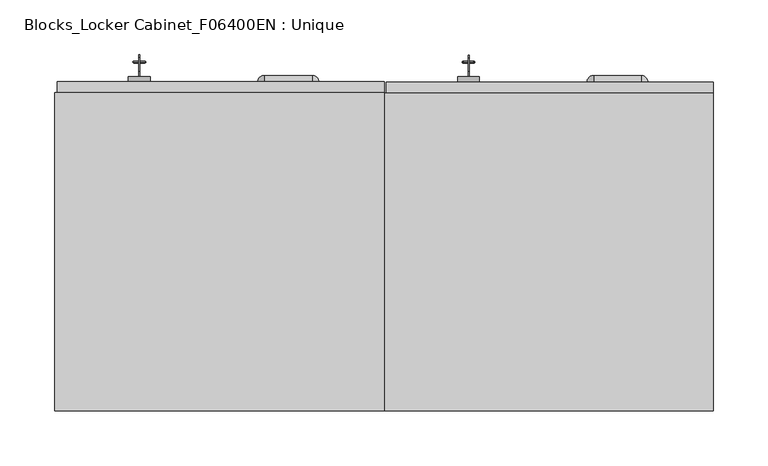
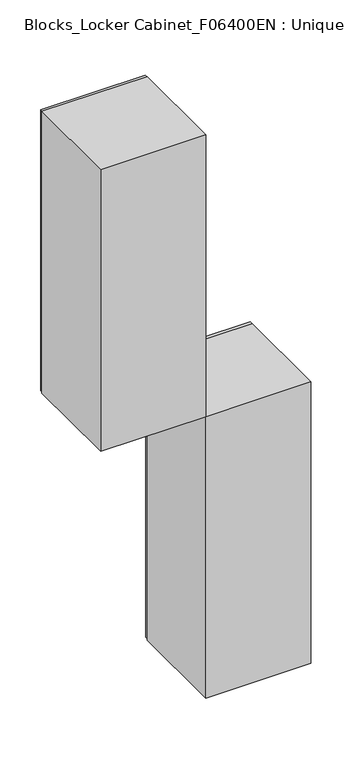
"""IFC4 building model written with IfcOpenShell, lengths in millimetres: furniture geometry, Blocks_Locker Cabinet_F06400EN : Unique."""

from ifc_helpers import new_model, si_unit, point, frame, frame_2d, origin, place, context, project, spatial, polyline, circle_curve, ellipse_curve, trimmed, segment, composite_curve, outline, extrude, faceted_brep, source, transform, mapped, element, save
from ifc_brep_helpers import plane_surface, cylinder_surface, revolved_surface, advanced_brep


def blocks_locker_cabinet_f06400en_unique_48c8ac53(model_context):
    return source(origin(), model_context, "Body", "SolidModel", [
        advanced_brep(
        [(-383.0, 12.5, 1375.0), (-363.0, 12.5, 1375.0), (-371.1588195, 12.5, 1382.0962926), (-374.8411805, 12.5, 1382.0962926), (-374.8411805, 12.5, 1372.8618188), (-371.1588195, 12.5, 1372.8618188), (-383.0, 7.5, 1375.0), (-363.0, 7.5, 1375.0), (-363.0, 10.7450625, 1375.0), (-383.0, 10.7450625, 1375.0), (-371.1588195, 10.7450625, 1372.8618188), (-371.1588195, 10.7450625, 1382.0962926), (-374.8411805, 10.7450625, 1372.8618188), (-374.8411805, 10.7450625, 1382.0962926)],
        [
            (0, 1, circle_curve(frame((-373.0, 12.5, 1375.0), z_axis=(0.0, 1.0, 0.0), x_axis=(1.0, 0.0, 0.0)), 10.0)),
            (1, 0, circle_curve(frame((-373.0, 12.5, 1375.0), z_axis=(0.0, 1.0, 0.0), x_axis=(1.0, 0.0, 0.0)), 10.0)),
            (2, 3),
            (3, 4),
            (4, 5),
            (5, 2),
            (6, 7, circle_curve(frame((-373.0, 7.5, 1375.0), z_axis=(0.0, -1.0, 0.0), x_axis=(1.0, 0.0, 0.0)), 10.0)),
            (7, 6, circle_curve(frame((-373.0, 7.5, 1375.0), z_axis=(0.0, -1.0, 0.0), x_axis=(1.0, 0.0, 0.0)), 10.0)),
            (1, 8),
            (8, 7),
            (6, 9),
            (9, 0),
            (5, 10),
            (10, 11),
            (11, 2),
            (4, 12),
            (12, 10),
            (3, 13),
            (13, 12),
            (11, 13),
        ],
        [
            plane_surface(frame((-363.0, 12.5, 1375.0), z_axis=(0.0, 1.0, 0.0), x_axis=(0.0, 0.0, 1.0))),
            plane_surface(frame((-363.0, 7.5, 1375.0), z_axis=(0.0, -1.0, 0.0), x_axis=(0.0, 0.0, -1.0))),
            cylinder_surface(frame((-373.0, 7.5, 1375.0), z_axis=(0.0, 1.0, 0.0), x_axis=(1.0, 0.0, 0.0)), 10.0),
            plane_surface(frame((-371.1588195, 12.5, 1382.0962926), z_axis=(-1.0, 0.0, 0.0), x_axis=(0.0, -1.0, 0.0))),
            plane_surface(frame((-371.1588195, 12.5, 1372.8618188), z_axis=(0.0, 0.0, 1.0), x_axis=(0.0, -1.0, 0.0))),
            plane_surface(frame((-374.8411805, 12.5, 1372.8618188), z_axis=(1.0, 0.0, 0.0), x_axis=(0.0, -1.0, 0.0))),
            plane_surface(frame((-374.8411805, 12.5, 1382.0962926), z_axis=(0.0, 0.0, -1.0), x_axis=(0.0, -1.0, 0.0))),
            plane_surface(frame((-363.0, 10.7450625, 1375.0), z_axis=(0.0, 1.0, 0.0), x_axis=(0.0, 0.0, 1.0))),
        ],
        [
            (0, [[1, 2], [3, 4, 5, 6]]),
            (1, [[7, 8]]),
            (2, [[9, 10, -7, 11, 12, -2]]),
            (2, [[-12, -11, -8, -10, -9, -1]]),
            (3, [[13, 14, 15, -6]]),
            (4, [[16, 17, -13, -5]]),
            (5, [[18, 19, -16, -4]]),
            (6, [[-15, 20, -18, -3]]),
            (7, [[-17, -19, -20, -14]]),
        ],
    ),
        extrude(outline(composite_curve([segment(polyline([(16.8246351, 1372.8618188), (13.7848488, 1372.8618188)]), True, "CONTINUOUS"), segment(trimmed(circle_curve(frame_2d((12.908516, 1372.8618188)), 0.8763328), [point((13.7848488, 1372.8618188))], [point((12.0321832, 1372.8618188))], True, "CARTESIAN"), True, "CONTINUOUS"), segment(polyline([(12.0321832, 1372.8618188), (10.7450625, 1372.8618188), (10.7450625, 1377.6669902), (17.0336838, 1377.6669902)]), True, "CONTINUOUS"), segment(trimmed(circle_curve(frame_2d((23.0067332, 1375.0)), 6.5414185), [point((17.0336838, 1377.6669902))], [point((16.8246351, 1372.8618188))], False, "CARTESIAN"), True, "CONTINUOUS")], self_intersect=False), holes=[composite_curve([segment(trimmed(circle_curve(frame_2d((25.6281997, 1375.0)), 1.688217), [point((27.3164167, 1375.0))], [point((23.9399827, 1375.0))], True, "CARTESIAN"), True, "CONTINUOUS"), segment(trimmed(circle_curve(frame_2d((25.6281997, 1375.0)), 1.688217), [point((23.9399827, 1375.0))], [point((27.3164167, 1375.0))], True, "CARTESIAN"), True, "CONTINUOUS")], self_intersect=False)]), frame((-373.4043078, 0.0, 0.0), z_axis=(1.0, 0.0, 0.0), x_axis=(0.0, 1.0, 0.0)), (0.0, 0.0, 1.0), 0.9157402),
        extrude(outline(composite_curve([segment(polyline([(27.8125, 1354.8018875), (27.8125, 1351.7621012)]), True, "CONTINUOUS"), segment(trimmed(circle_curve(frame_2d((27.8125, 1350.8857684)), 0.8763328), [point((27.8125, 1351.7621012))], [point((27.8125, 1350.0094356))], True, "CARTESIAN"), True, "CONTINUOUS"), segment(polyline([(27.8125, 1350.0094356), (27.8125, 1347.7621012)]), True, "CONTINUOUS"), segment(trimmed(circle_curve(frame_2d((27.8125, 1346.8857684)), 0.8763328), [point((27.8125, 1347.7621012))], [point((27.8125, 1346.0094356))], True, "CARTESIAN"), True, "CONTINUOUS"), segment(polyline([(27.8125, 1346.0094356), (27.8125, 1343.7621012)]), True, "CONTINUOUS"), segment(trimmed(circle_curve(frame_2d((27.8125, 1342.8857684)), 0.8763328), [point((27.8125, 1343.7621012))], [point((27.8125, 1342.0094356))], True, "CARTESIAN"), True, "CONTINUOUS"), segment(polyline([(27.8125, 1342.0094356), (27.8125, 1340.3532579), (25.9613419, 1337.7095301), (24.2573286, 1337.7095301), (24.2573286, 1354.5978839)]), True, "CONTINUOUS"), segment(trimmed(circle_curve(frame_2d((25.6743188, 1360.9839856)), 6.5414185), [point((24.2573286, 1354.5978839))], [point((27.8125, 1354.8018875))], False, "CARTESIAN"), True, "CONTINUOUS")], self_intersect=False), holes=[composite_curve([segment(trimmed(circle_curve(frame_2d((25.6743188, 1363.6054521)), 1.688217), [point((25.6743188, 1365.2936691))], [point((25.6743188, 1361.9172351))], True, "CARTESIAN"), True, "CONTINUOUS"), segment(trimmed(circle_curve(frame_2d((25.6743188, 1363.6054521)), 1.688217), [point((25.6743188, 1361.9172351))], [point((25.6743188, 1365.2936691))], True, "CARTESIAN"), True, "CONTINUOUS")], self_intersect=False)]), frame((-373.4043078, 0.0, 0.0), z_axis=(1.0, 0.0, 0.0), x_axis=(0.0, 1.0, 0.0)), (0.0, 0.0, 1.0), 0.9157402),
        advanced_brep(
        [(-368.8, 25.663019, 1369.4000012), (-367.2, 25.663019, 1369.4000012), (-378.8, 25.663019, 1369.4000012), (-377.2, 25.663019, 1369.4000012)],
        [
            (0, 1, circle_curve(frame((-368.0, 25.663019, 1369.4000012), z_axis=(0.0, 0.0, -1.0), x_axis=(-1.0, 0.0, 0.0)), 0.8)),
            (1, 2, circle_curve(frame((-373.0, 25.663019, 1369.4000012), z_axis=(0.0, 1.0, 0.0), x_axis=(-1.0, 0.0, 0.0)), 5.8)),
            (2, 3, circle_curve(frame((-378.0, 25.663019, 1369.4000012), z_axis=(0.0, 0.0, -1.0), x_axis=(1.0, 0.0, 0.0)), 0.8)),
            (3, 0, circle_curve(frame((-373.0, 25.663019, 1369.4000012), z_axis=(0.0, -1.0, 0.0), x_axis=(-1.0, 0.0, 0.0)), 4.2)),
            (1, 0, circle_curve(frame((-368.0, 25.663019, 1369.4000012), z_axis=(0.0, 0.0, -1.0), x_axis=(-1.0, 0.0, 0.0)), 0.8)),
            (3, 2, circle_curve(frame((-378.0, 25.663019, 1369.4000012), z_axis=(0.0, 0.0, -1.0), x_axis=(1.0, 0.0, 0.0)), 0.8)),
            (2, 1, circle_curve(frame((-373.0, 25.663019, 1369.4000012), z_axis=(0.0, 1.0, 0.0), x_axis=(1.0, 0.0, 0.0)), 5.8)),
            (0, 3, circle_curve(frame((-373.0, 25.663019, 1369.4000012), z_axis=(0.0, -1.0, 0.0), x_axis=(1.0, 0.0, 0.0)), 4.2)),
        ],
        [
            revolved_surface(trimmed(ellipse_curve(frame((-378.0, 25.663019, 1369.4000012), z_axis=(0.0, 0.0, -1.0), x_axis=(1.0, 0.0, 0.0)), 0.8, 0.8), [point((-378.8, 25.663019, 1369.4000012))], [point((-377.2, 25.663019, 1369.4000012))], True, "CARTESIAN"), (-373.0, -2.5, 1369.4000012), (0.0, 1.0, 0.0)),
            revolved_surface(trimmed(ellipse_curve(frame((-378.0, 25.663019, 1369.4000012), z_axis=(0.0, 0.0, -1.0), x_axis=(1.0, 0.0, 0.0)), 0.8, 0.8), [point((-377.2, 25.663019, 1369.4000012))], [point((-378.8, 25.663019, 1369.4000012))], True, "CARTESIAN"), (-373.0, -2.5, 1369.4000012), (0.0, 1.0, 0.0)),
            revolved_surface(trimmed(ellipse_curve(frame((-368.0, 25.663019, 1369.4000012), z_axis=(0.0, 0.0, 1.0), x_axis=(-1.0, 0.0, 0.0)), 0.8, 0.8), [point((-367.2, 25.663019, 1369.4000012))], [point((-368.8, 25.663019, 1369.4000012))], True, "CARTESIAN"), (-373.0, -2.5, 1369.4000012), (0.0, 1.0, 0.0)),
            revolved_surface(trimmed(ellipse_curve(frame((-368.0, 25.663019, 1369.4000012), z_axis=(0.0, 0.0, 1.0), x_axis=(-1.0, 0.0, 0.0)), 0.8, 0.8), [point((-368.8, 25.663019, 1369.4000012))], [point((-367.2, 25.663019, 1369.4000012))], True, "CARTESIAN"), (-373.0, -2.5, 1369.4000012), (0.0, 1.0, 0.0)),
        ],
        [
            (0, [[1, 2, 3, 4]]),
            (1, [[5, -4, 6, -2]]),
            (2, [[-3, 7, -1, 8]]),
            (3, [[-6, -8, -5, -7]]),
        ],
    ),
        advanced_brep(
        [(-448.0, 7.5, 1799.0), (-448.0, -2.5, 1799.0), (-150.0, -2.5, 1799.0), (-150.0, 7.5, 1799.0), (-448.0, 7.5, 951.0), (-150.0, 7.5, 951.0), (-150.0, -2.5, 951.0), (-448.0, -2.5, 951.0), (-393.0, 7.5, 1525.0), (-393.0, 7.5, 1405.0), (-333.7890736, 7.5, 1405.0), (-333.7890736, 7.5, 1525.0), (-380.6526901, 0.3712773, 1525.0), (-357.2105549, 3.975278, 1525.0), (-380.6526901, 0.3712773, 1405.0), (-357.2105549, 3.975278, 1405.0)],
        [
            (0, 1),
            (1, 2),
            (2, 3),
            (3, 0),
            (4, 5),
            (5, 6),
            (6, 7),
            (7, 4),
            (3, 5),
            (4, 0),
            (8, 9),
            (9, 10),
            (10, 11),
            (11, 8),
            (2, 6),
            (1, 7),
            (12, 8),
            (11, 13),
            (13, 12, circle_curve(frame((-371.1776523, 16.7825242, 1525.0), z_axis=(0.0, 0.0, -1.0), x_axis=(0.0, 1.0, 0.0)), 18.9500756)),
            (14, 15, circle_curve(frame((-371.1776523, 16.7825242, 1405.0), z_axis=(0.0, 0.0, 1.0), x_axis=(0.0, 1.0, 0.0)), 18.9500756)),
            (15, 10),
            (9, 14),
            (12, 14),
            (15, 13),
        ],
        [
            plane_surface(frame((-150.0, 7.5, 1799.0), z_axis=(0.0, 0.0, 1.0), x_axis=(1.0, 0.0, 0.0))),
            plane_surface(frame((-150.0, 7.5, 951.0), z_axis=(0.0, 0.0, -1.0), x_axis=(-1.0, 0.0, 0.0))),
            plane_surface(frame((-448.0, 7.5, 1799.0), z_axis=(0.0, 1.0, 0.0), x_axis=(0.0, 0.0, -1.0))),
            plane_surface(frame((-150.0, 7.5, 1799.0), z_axis=(1.0, 0.0, 0.0), x_axis=(0.0, 0.0, -1.0))),
            plane_surface(frame((-150.0, -2.5, 1799.0), z_axis=(0.0, -1.0, 0.0), x_axis=(0.0, 0.0, -1.0))),
            plane_surface(frame((-448.0, -2.5, 1799.0), z_axis=(-1.0, 0.0, 0.0), x_axis=(0.0, 0.0, -1.0))),
            plane_surface(frame((-393.0, 7.5, 1525.0), z_axis=(0.0, 0.0, -1.0), x_axis=(-0.866025403784437, 0.5000000000000028, 0.0))),
            plane_surface(frame((-393.0, 7.5, 1405.0), z_axis=(0.0, 0.0, 1.0), x_axis=(0.866025403784437, -0.5000000000000028, 0.0))),
            plane_surface(frame((-380.6526901, 0.3712773, 1525.0), z_axis=(0.5000000000000028, 0.866025403784437, 0.0), x_axis=(0.0, 0.0, -1.0))),
            plane_surface(frame((-333.7890736, 7.5, 1525.0), z_axis=(-0.14881527984319862, 0.9888650122666847, 0.0), x_axis=(0.0, 0.0, -1.0))),
            revolved_surface(polyline([(-371.1776523, 35.7325998, 1525.0), (-371.1776523, 35.7325998, 1405.0)]), (-371.1776523, 16.7825242, 1405.0), (0.0, 0.0, 1.0)),
        ],
        [
            (0, [[1, 2, 3, 4]]),
            (1, [[5, 6, 7, 8]]),
            (2, [[9, -5, 10, -4], [11, 12, 13, 14]]),
            (3, [[15, -6, -9, -3]]),
            (4, [[16, -7, -15, -2]]),
            (5, [[-10, -8, -16, -1]]),
            (6, [[17, -14, 18, 19]]),
            (7, [[20, 21, -12, 22]]),
            (8, [[23, -22, -11, -17]]),
            (9, [[-13, -21, 24, -18]]),
            (10, [[-24, -20, -23, -19]]),
        ],
    ),
        advanced_brep(
        [(-265.0, 7.5, 991.0), (-209.4810333, 7.5, 991.0), (-215.4810333, 7.5, 997.0), (-259.0, 7.5, 997.0), (-259.0, 13.5, 991.0), (-215.4810333, 13.5, 991.0)],
        [
            (0, 1),
            (1, 2, circle_curve(frame((-215.4810333, 7.5, 991.0), z_axis=(0.0, -1.0, 0.0), x_axis=(1.0, 0.0, 0.0)), 6.0)),
            (2, 3),
            (3, 0, circle_curve(frame((-259.0, 7.5, 991.0), z_axis=(0.0, -1.0, 0.0), x_axis=(1.0, 0.0, 0.0)), 6.0)),
            (0, 4, circle_curve(frame((-259.0, 7.5, 991.0), z_axis=(0.0, 0.0, -1.0), x_axis=(1.0, 0.0, 0.0)), 6.0)),
            (4, 5),
            (5, 1, circle_curve(frame((-215.4810333, 7.5, 991.0), z_axis=(0.0, 0.0, -1.0), x_axis=(1.0, 0.0, 0.0)), 6.0)),
            (3, 4, circle_curve(frame((-259.0, 7.5, 991.0), z_axis=(-1.0, 0.0, 0.0), x_axis=(0.0, 0.0, 1.0)), 6.0)),
            (2, 5, circle_curve(frame((-215.4810333, 7.5, 991.0), z_axis=(-1.0, 0.0, 0.0), x_axis=(0.0, 0.0, 1.0)), 6.0)),
        ],
        [
            plane_surface(frame((-215.0, 7.5, 991.0), z_axis=(0.0, -1.0, 0.0), x_axis=(0.0, 0.0, 1.0))),
            plane_surface(frame((-215.0, 7.5, 991.0), z_axis=(0.0, 0.0, -1.0), x_axis=(0.0, 1.0, 0.0))),
            revolved_surface(trimmed(ellipse_curve(frame((-259.0, 7.5, 991.0), z_axis=(0.0, 1.0, 0.0), x_axis=(1.0, 0.0, 0.0)), 6.0, 6.0), [point((-265.0, 7.5, 991.0))], [point((-259.0, 7.5, 997.0))], True, "CARTESIAN"), (-215.0, 7.5, 991.0), (1.0, 0.0, 0.0)),
            cylinder_surface(frame((-215.0, 7.5, 991.0), z_axis=(1.0, 0.0, 0.0), x_axis=(0.0, 0.0, 1.0)), 6.0),
            revolved_surface(trimmed(ellipse_curve(frame((-215.4810333, 7.5, 991.0), z_axis=(0.0, 1.0, 0.0), x_axis=(1.0, 0.0, 0.0)), 6.0, 6.0), [point((-215.4810333, 7.5, 997.0))], [point((-209.4810333, 7.5, 991.0))], True, "CARTESIAN"), (-215.0, 7.5, 991.0), (1.0, 0.0, 0.0)),
        ],
        [
            (0, [[1, 2, 3, 4]]),
            (1, [[-1, 5, 6, 7]]),
            (2, [[-5, -4, 8]]),
            (3, [[-6, -8, -3, 9]]),
            (4, [[-7, -9, -2]]),
        ],
    ),
        advanced_brep(
        [(-265.0, 7.5, 1006.0), (-209.4810333, 7.5, 1006.0), (-215.4810333, 7.5, 1012.0), (-259.0, 7.5, 1012.0), (-259.0, 13.5, 1006.0), (-215.4810333, 13.5, 1006.0)],
        [
            (0, 1),
            (1, 2, circle_curve(frame((-215.4810333, 7.5, 1006.0), z_axis=(0.0, -1.0, 0.0), x_axis=(1.0, 0.0, 0.0)), 6.0)),
            (2, 3),
            (3, 0, circle_curve(frame((-259.0, 7.5, 1006.0), z_axis=(0.0, -1.0, 0.0), x_axis=(1.0, 0.0, 0.0)), 6.0)),
            (0, 4, circle_curve(frame((-259.0, 7.5, 1006.0), z_axis=(0.0, 0.0, -1.0), x_axis=(1.0, 0.0, 0.0)), 6.0)),
            (4, 5),
            (5, 1, circle_curve(frame((-215.4810333, 7.5, 1006.0), z_axis=(0.0, 0.0, -1.0), x_axis=(1.0, 0.0, 0.0)), 6.0)),
            (3, 4, circle_curve(frame((-259.0, 7.5, 1006.0), z_axis=(-1.0, 0.0, 0.0), x_axis=(0.0, 0.0, 1.0)), 6.0)),
            (2, 5, circle_curve(frame((-215.4810333, 7.5, 1006.0), z_axis=(-1.0, 0.0, 0.0), x_axis=(0.0, 0.0, 1.0)), 6.0)),
        ],
        [
            plane_surface(frame((-215.0, 7.5, 1006.0), z_axis=(0.0, -1.0, 0.0), x_axis=(0.0, 0.0, 1.0))),
            plane_surface(frame((-215.0, 7.5, 1006.0), z_axis=(0.0, 0.0, -1.0), x_axis=(0.0, 1.0, 0.0))),
            revolved_surface(trimmed(ellipse_curve(frame((-259.0, 7.5, 1006.0), z_axis=(0.0, 1.0, 0.0), x_axis=(1.0, 0.0, 0.0)), 6.0, 6.0), [point((-265.0, 7.5, 1006.0))], [point((-259.0, 7.5, 1012.0))], True, "CARTESIAN"), (-215.0, 7.5, 1006.0), (1.0, 0.0, 0.0)),
            cylinder_surface(frame((-215.0, 7.5, 1006.0), z_axis=(1.0, 0.0, 0.0), x_axis=(0.0, 0.0, 1.0)), 6.0),
            revolved_surface(trimmed(ellipse_curve(frame((-215.4810333, 7.5, 1006.0), z_axis=(0.0, 1.0, 0.0), x_axis=(1.0, 0.0, 0.0)), 6.0, 6.0), [point((-215.4810333, 7.5, 1012.0))], [point((-209.4810333, 7.5, 1006.0))], True, "CARTESIAN"), (-215.0, 7.5, 1006.0), (1.0, 0.0, 0.0)),
        ],
        [
            (0, [[1, 2, 3, 4]]),
            (1, [[-1, 5, 6, 7]]),
            (2, [[-5, -4, 8]]),
            (3, [[-6, -8, -3, 9]]),
            (4, [[-7, -9, -2]]),
        ],
    ),
        advanced_brep(
        [(-265.0, 7.5, 1021.0), (-209.4810333, 7.5, 1021.0), (-215.4810333, 7.5, 1027.0), (-259.0, 7.5, 1027.0), (-259.0, 13.5, 1021.0), (-215.4810333, 13.5, 1021.0)],
        [
            (0, 1),
            (1, 2, circle_curve(frame((-215.4810333, 7.5, 1021.0), z_axis=(0.0, -1.0, 0.0), x_axis=(1.0, 0.0, 0.0)), 6.0)),
            (2, 3),
            (3, 0, circle_curve(frame((-259.0, 7.5, 1021.0), z_axis=(0.0, -1.0, 0.0), x_axis=(1.0, 0.0, 0.0)), 6.0)),
            (0, 4, circle_curve(frame((-259.0, 7.5, 1021.0), z_axis=(0.0, 0.0, -1.0), x_axis=(1.0, 0.0, 0.0)), 6.0)),
            (4, 5),
            (5, 1, circle_curve(frame((-215.4810333, 7.5, 1021.0), z_axis=(0.0, 0.0, -1.0), x_axis=(1.0, 0.0, 0.0)), 6.0)),
            (3, 4, circle_curve(frame((-259.0, 7.5, 1021.0), z_axis=(-1.0, 0.0, 0.0), x_axis=(0.0, 0.0, 1.0)), 6.0)),
            (2, 5, circle_curve(frame((-215.4810333, 7.5, 1021.0), z_axis=(-1.0, 0.0, 0.0), x_axis=(0.0, 0.0, 1.0)), 6.0)),
        ],
        [
            plane_surface(frame((-215.0, 7.5, 1021.0), z_axis=(0.0, -1.0, 0.0), x_axis=(0.0, 0.0, 1.0))),
            plane_surface(frame((-215.0, 7.5, 1021.0), z_axis=(0.0, 0.0, -1.0), x_axis=(0.0, 1.0, 0.0))),
            revolved_surface(trimmed(ellipse_curve(frame((-259.0, 7.5, 1021.0), z_axis=(0.0, 1.0, 0.0), x_axis=(1.0, 0.0, 0.0)), 6.0, 6.0), [point((-265.0, 7.5, 1021.0))], [point((-259.0, 7.5, 1027.0))], True, "CARTESIAN"), (-215.0, 7.5, 1021.0), (1.0, 0.0, 0.0)),
            cylinder_surface(frame((-215.0, 7.5, 1021.0), z_axis=(1.0, 0.0, 0.0), x_axis=(0.0, 0.0, 1.0)), 6.0),
            revolved_surface(trimmed(ellipse_curve(frame((-215.4810333, 7.5, 1021.0), z_axis=(0.0, 1.0, 0.0), x_axis=(1.0, 0.0, 0.0)), 6.0, 6.0), [point((-215.4810333, 7.5, 1027.0))], [point((-209.4810333, 7.5, 1021.0))], True, "CARTESIAN"), (-215.0, 7.5, 1021.0), (1.0, 0.0, 0.0)),
        ],
        [
            (0, [[1, 2, 3, 4]]),
            (1, [[-1, 5, 6, 7]]),
            (2, [[-5, -4, 8]]),
            (3, [[-6, -8, -3, 9]]),
            (4, [[-7, -9, -2]]),
        ],
    ),
        advanced_brep(
        [(-265.0, 7.5, 1036.0), (-209.4810333, 7.5, 1036.0), (-215.4810333, 7.5, 1042.0), (-259.0, 7.5, 1042.0), (-259.0, 13.5, 1036.0), (-215.4810333, 13.5, 1036.0)],
        [
            (0, 1),
            (1, 2, circle_curve(frame((-215.4810333, 7.5, 1036.0), z_axis=(0.0, -1.0, 0.0), x_axis=(1.0, 0.0, 0.0)), 6.0)),
            (2, 3),
            (3, 0, circle_curve(frame((-259.0, 7.5, 1036.0), z_axis=(0.0, -1.0, 0.0), x_axis=(1.0, 0.0, 0.0)), 6.0)),
            (0, 4, circle_curve(frame((-259.0, 7.5, 1036.0), z_axis=(0.0, 0.0, -1.0), x_axis=(1.0, 0.0, 0.0)), 6.0)),
            (4, 5),
            (5, 1, circle_curve(frame((-215.4810333, 7.5, 1036.0), z_axis=(0.0, 0.0, -1.0), x_axis=(1.0, 0.0, 0.0)), 6.0)),
            (3, 4, circle_curve(frame((-259.0, 7.5, 1036.0), z_axis=(-1.0, 0.0, 0.0), x_axis=(0.0, 0.0, 1.0)), 6.0)),
            (2, 5, circle_curve(frame((-215.4810333, 7.5, 1036.0), z_axis=(-1.0, 0.0, 0.0), x_axis=(0.0, 0.0, 1.0)), 6.0)),
        ],
        [
            plane_surface(frame((-215.0, 7.5, 1036.0), z_axis=(0.0, -1.0, 0.0), x_axis=(0.0, 0.0, 1.0))),
            plane_surface(frame((-215.0, 7.5, 1036.0), z_axis=(0.0, 0.0, -1.0), x_axis=(0.0, 1.0, 0.0))),
            revolved_surface(trimmed(ellipse_curve(frame((-259.0, 7.5, 1036.0), z_axis=(0.0, 1.0, 0.0), x_axis=(1.0, 0.0, 0.0)), 6.0, 6.0), [point((-265.0, 7.5, 1036.0))], [point((-259.0, 7.5, 1042.0))], True, "CARTESIAN"), (-215.0, 7.5, 1036.0), (1.0, 0.0, 0.0)),
            cylinder_surface(frame((-215.0, 7.5, 1036.0), z_axis=(1.0, 0.0, 0.0), x_axis=(0.0, 0.0, 1.0)), 6.0),
            revolved_surface(trimmed(ellipse_curve(frame((-215.4810333, 7.5, 1036.0), z_axis=(0.0, 1.0, 0.0), x_axis=(1.0, 0.0, 0.0)), 6.0, 6.0), [point((-215.4810333, 7.5, 1042.0))], [point((-209.4810333, 7.5, 1036.0))], True, "CARTESIAN"), (-215.0, 7.5, 1036.0), (1.0, 0.0, 0.0)),
        ],
        [
            (0, [[1, 2, 3, 4]]),
            (1, [[-1, 5, 6, 7]]),
            (2, [[-5, -4, 8]]),
            (3, [[-6, -8, -3, 9]]),
            (4, [[-7, -9, -2]]),
        ],
    ),
        advanced_brep(
        [(-265.0, 7.5, 1051.0), (-209.4810333, 7.5, 1051.0), (-215.4810333, 7.5, 1057.0), (-259.0, 7.5, 1057.0), (-259.0, 13.5, 1051.0), (-215.4810333, 13.5, 1051.0)],
        [
            (0, 1),
            (1, 2, circle_curve(frame((-215.4810333, 7.5, 1051.0), z_axis=(0.0, -1.0, 0.0), x_axis=(1.0, 0.0, 0.0)), 6.0)),
            (2, 3),
            (3, 0, circle_curve(frame((-259.0, 7.5, 1051.0), z_axis=(0.0, -1.0, 0.0), x_axis=(1.0, 0.0, 0.0)), 6.0)),
            (0, 4, circle_curve(frame((-259.0, 7.5, 1051.0), z_axis=(0.0, 0.0, -1.0), x_axis=(1.0, 0.0, 0.0)), 6.0)),
            (4, 5),
            (5, 1, circle_curve(frame((-215.4810333, 7.5, 1051.0), z_axis=(0.0, 0.0, -1.0), x_axis=(1.0, 0.0, 0.0)), 6.0)),
            (3, 4, circle_curve(frame((-259.0, 7.5, 1051.0), z_axis=(-1.0, 0.0, 0.0), x_axis=(0.0, 0.0, 1.0)), 6.0)),
            (2, 5, circle_curve(frame((-215.4810333, 7.5, 1051.0), z_axis=(-1.0, 0.0, 0.0), x_axis=(0.0, 0.0, 1.0)), 6.0)),
        ],
        [
            plane_surface(frame((-215.0, 7.5, 1051.0), z_axis=(0.0, -1.0, 0.0), x_axis=(0.0, 0.0, 1.0))),
            plane_surface(frame((-215.0, 7.5, 1051.0), z_axis=(0.0, 0.0, -1.0), x_axis=(0.0, 1.0, 0.0))),
            revolved_surface(trimmed(ellipse_curve(frame((-259.0, 7.5, 1051.0), z_axis=(0.0, 1.0, 0.0), x_axis=(1.0, 0.0, 0.0)), 6.0, 6.0), [point((-265.0, 7.5, 1051.0))], [point((-259.0, 7.5, 1057.0))], True, "CARTESIAN"), (-215.0, 7.5, 1051.0), (1.0, 0.0, 0.0)),
            cylinder_surface(frame((-215.0, 7.5, 1051.0), z_axis=(1.0, 0.0, 0.0), x_axis=(0.0, 0.0, 1.0)), 6.0),
            revolved_surface(trimmed(ellipse_curve(frame((-215.4810333, 7.5, 1051.0), z_axis=(0.0, 1.0, 0.0), x_axis=(1.0, 0.0, 0.0)), 6.0, 6.0), [point((-215.4810333, 7.5, 1057.0))], [point((-209.4810333, 7.5, 1051.0))], True, "CARTESIAN"), (-215.0, 7.5, 1051.0), (1.0, 0.0, 0.0)),
        ],
        [
            (0, [[1, 2, 3, 4]]),
            (1, [[-1, 5, 6, 7]]),
            (2, [[-5, -4, 8]]),
            (3, [[-6, -8, -3, 9]]),
            (4, [[-7, -9, -2]]),
        ],
    ),
        extrude(outline(composite_curve([segment(polyline([(-380.6526901, 0.3712773), (-393.0, 7.5), (-333.7890736, 7.5), (-357.2105549, 3.975278)]), True, "CONTINUOUS"), segment(trimmed(circle_curve(frame_2d((-371.1776523, 16.7825242)), 18.9500756), [point((-357.2105549, 3.975278))], [point((-380.6526901, 0.3712773))], False, "CARTESIAN"), True, "CONTINUOUS")], self_intersect=False)), frame((0.0, 0.0, 1405.0), z_axis=(0.0, 0.0, 1.0), x_axis=(1.0, 0.0, 0.0)), (0.0, 0.0, 1.0), 5.0),
        extrude(outline(composite_curve([segment(polyline([(-380.6526901, 0.3712773), (-393.0, 7.5), (-333.7890736, 7.5), (-357.2105549, 3.975278)]), True, "CONTINUOUS"), segment(trimmed(circle_curve(frame_2d((-371.1776523, 16.7825242)), 18.9500756), [point((-357.2105549, 3.975278))], [point((-380.6526901, 0.3712773))], False, "CARTESIAN"), True, "CONTINUOUS")], self_intersect=False)), frame((0.0, 0.0, 1520.0), z_axis=(0.0, 0.0, 1.0), x_axis=(1.0, 0.0, 0.0)), (0.0, 0.0, 1.0), 5.0),
        faceted_brep([(-150.0, -2.5, 1800.0), (-150.0, -2.5, 950.0), (-450.0, -2.5, 950.0), (-450.0, -2.5, 1800.0), (-160.0, -2.5, 1790.0), (-440.0, -2.5, 1790.0), (-440.0, -2.5, 960.0), (-160.0, -2.5, 960.0), (-150.0, -292.5, 1800.0), (-450.0, -292.5, 1800.0), (-450.0, -292.5, 950.0), (-150.0, -292.5, 950.0), (-450.0, -282.5, 1800.0), (-150.0, -282.5, 1800.0), (-450.0, -282.5, 950.0), (-150.0, -282.5, 950.0), (-160.0, -282.5, 960.0), (-160.0, -282.5, 1790.0), (-440.0, -282.5, 960.0), (-440.0, -282.5, 1790.0)], [[[0, 1, 2, 3], [4, 5, 6, 7]], [[8, 9, 10, 11]], [[3, 12, 9, 8, 13, 0]], [[2, 14, 10, 9, 12, 3]], [[1, 15, 11, 10, 14, 2]], [[0, 13, 8, 11, 15, 1]], [[7, 16, 17, 4]], [[6, 18, 16, 7]], [[5, 19, 18, 6]], [[4, 17, 19, 5]], [[16, 18, 19, 17]]]),
        advanced_brep(
        [(-83.0, 12.5, 525.0), (-63.0, 12.5, 525.0), (-71.1588195, 12.5, 532.0962926), (-74.8411805, 12.5, 532.0962926), (-74.8411805, 12.5, 522.8618188), (-71.1588195, 12.5, 522.8618188), (-83.0, 7.5, 525.0), (-63.0, 7.5, 525.0), (-63.0, 10.7450625, 525.0), (-83.0, 10.7450625, 525.0), (-71.1588195, 10.7450625, 522.8618188), (-71.1588195, 10.7450625, 532.0962926), (-74.8411805, 10.7450625, 522.8618188), (-74.8411805, 10.7450625, 532.0962926)],
        [
            (0, 1, circle_curve(frame((-73.0, 12.5, 525.0), z_axis=(0.0, 1.0, 0.0), x_axis=(1.0, 0.0, 0.0)), 10.0)),
            (1, 0, circle_curve(frame((-73.0, 12.5, 525.0), z_axis=(0.0, 1.0, 0.0), x_axis=(1.0, 0.0, 0.0)), 10.0)),
            (2, 3),
            (3, 4),
            (4, 5),
            (5, 2),
            (6, 7, circle_curve(frame((-73.0, 7.5, 525.0), z_axis=(0.0, -1.0, 0.0), x_axis=(1.0, 0.0, 0.0)), 10.0)),
            (7, 6, circle_curve(frame((-73.0, 7.5, 525.0), z_axis=(0.0, -1.0, 0.0), x_axis=(1.0, 0.0, 0.0)), 10.0)),
            (1, 8),
            (8, 7),
            (6, 9),
            (9, 0),
            (5, 10),
            (10, 11),
            (11, 2),
            (4, 12),
            (12, 10),
            (3, 13),
            (13, 12),
            (11, 13),
        ],
        [
            plane_surface(frame((-63.0, 12.5, 525.0), z_axis=(0.0, 1.0, 0.0), x_axis=(0.0, 0.0, 1.0))),
            plane_surface(frame((-63.0, 7.5, 525.0), z_axis=(0.0, -1.0, 0.0), x_axis=(0.0, 0.0, -1.0))),
            cylinder_surface(frame((-73.0, 7.5, 525.0), z_axis=(0.0, 1.0, 0.0), x_axis=(1.0, 0.0, 0.0)), 10.0),
            plane_surface(frame((-71.1588195, 12.5, 532.0962926), z_axis=(-1.0, 0.0, 0.0), x_axis=(0.0, -1.0, 0.0))),
            plane_surface(frame((-71.1588195, 12.5, 522.8618188), z_axis=(0.0, 0.0, 1.0), x_axis=(0.0, -1.0, 0.0))),
            plane_surface(frame((-74.8411805, 12.5, 522.8618188), z_axis=(1.0, 0.0, 0.0), x_axis=(0.0, -1.0, 0.0))),
            plane_surface(frame((-74.8411805, 12.5, 532.0962926), z_axis=(0.0, 0.0, -1.0), x_axis=(0.0, -1.0, 0.0))),
            plane_surface(frame((-63.0, 10.7450625, 525.0), z_axis=(0.0, 1.0, 0.0), x_axis=(0.0, 0.0, 1.0))),
        ],
        [
            (0, [[1, 2], [3, 4, 5, 6]]),
            (1, [[7, 8]]),
            (2, [[9, 10, -7, 11, 12, -2]]),
            (2, [[-12, -11, -8, -10, -9, -1]]),
            (3, [[13, 14, 15, -6]]),
            (4, [[16, 17, -13, -5]]),
            (5, [[18, 19, -16, -4]]),
            (6, [[-15, 20, -18, -3]]),
            (7, [[-17, -19, -20, -14]]),
        ],
    ),
        extrude(outline(composite_curve([segment(polyline([(16.8246351, 522.8618188), (13.7848488, 522.8618188)]), True, "CONTINUOUS"), segment(trimmed(circle_curve(frame_2d((12.908516, 522.8618188)), 0.8763328), [point((13.7848488, 522.8618188))], [point((12.0321832, 522.8618188))], True, "CARTESIAN"), True, "CONTINUOUS"), segment(polyline([(12.0321832, 522.8618188), (10.7450625, 522.8618188), (10.7450625, 527.6669902), (17.0336838, 527.6669902)]), True, "CONTINUOUS"), segment(trimmed(circle_curve(frame_2d((23.0067332, 525.0)), 6.5414185), [point((17.0336838, 527.6669902))], [point((16.8246351, 522.8618188))], False, "CARTESIAN"), True, "CONTINUOUS")], self_intersect=False), holes=[composite_curve([segment(trimmed(circle_curve(frame_2d((25.6281997, 525.0)), 1.688217), [point((27.3164167, 525.0))], [point((23.9399827, 525.0))], True, "CARTESIAN"), True, "CONTINUOUS"), segment(trimmed(circle_curve(frame_2d((25.6281997, 525.0)), 1.688217), [point((23.9399827, 525.0))], [point((27.3164167, 525.0))], True, "CARTESIAN"), True, "CONTINUOUS")], self_intersect=False)]), frame((-73.4043078, 0.0, 0.0), z_axis=(1.0, 0.0, 0.0), x_axis=(0.0, 1.0, 0.0)), (0.0, 0.0, 1.0), 0.9157402),
        extrude(outline(composite_curve([segment(polyline([(27.8125, 504.8018875), (27.8125, 501.7621012)]), True, "CONTINUOUS"), segment(trimmed(circle_curve(frame_2d((27.8125, 500.8857684)), 0.8763328), [point((27.8125, 501.7621012))], [point((27.8125, 500.0094356))], True, "CARTESIAN"), True, "CONTINUOUS"), segment(polyline([(27.8125, 500.0094356), (27.8125, 497.7621012)]), True, "CONTINUOUS"), segment(trimmed(circle_curve(frame_2d((27.8125, 496.8857684)), 0.8763328), [point((27.8125, 497.7621012))], [point((27.8125, 496.0094356))], True, "CARTESIAN"), True, "CONTINUOUS"), segment(polyline([(27.8125, 496.0094356), (27.8125, 493.7621012)]), True, "CONTINUOUS"), segment(trimmed(circle_curve(frame_2d((27.8125, 492.8857684)), 0.8763328), [point((27.8125, 493.7621012))], [point((27.8125, 492.0094356))], True, "CARTESIAN"), True, "CONTINUOUS"), segment(polyline([(27.8125, 492.0094356), (27.8125, 490.3532579), (25.9613419, 487.7095301), (24.2573286, 487.7095301), (24.2573286, 504.5978839)]), True, "CONTINUOUS"), segment(trimmed(circle_curve(frame_2d((25.6743188, 510.9839856)), 6.5414185), [point((24.2573286, 504.5978839))], [point((27.8125, 504.8018875))], False, "CARTESIAN"), True, "CONTINUOUS")], self_intersect=False), holes=[composite_curve([segment(trimmed(circle_curve(frame_2d((25.6743188, 513.6054521)), 1.688217), [point((25.6743188, 515.2936691))], [point((25.6743188, 511.9172351))], True, "CARTESIAN"), True, "CONTINUOUS"), segment(trimmed(circle_curve(frame_2d((25.6743188, 513.6054521)), 1.688217), [point((25.6743188, 511.9172351))], [point((25.6743188, 515.2936691))], True, "CARTESIAN"), True, "CONTINUOUS")], self_intersect=False)]), frame((-73.4043078, 0.0, 0.0), z_axis=(1.0, 0.0, 0.0), x_axis=(0.0, 1.0, 0.0)), (0.0, 0.0, 1.0), 0.9157402),
        advanced_brep(
        [(-68.8, 25.663019, 519.4000012), (-67.2, 25.663019, 519.4000012), (-78.8, 25.663019, 519.4000012), (-77.2, 25.663019, 519.4000012)],
        [
            (0, 1, circle_curve(frame((-68.0, 25.663019, 519.4000012), z_axis=(0.0, 0.0, -1.0), x_axis=(-1.0, 0.0, 0.0)), 0.8)),
            (1, 2, circle_curve(frame((-73.0, 25.663019, 519.4000012), z_axis=(0.0, 1.0, 0.0), x_axis=(-1.0, 0.0, 0.0)), 5.8)),
            (2, 3, circle_curve(frame((-78.0, 25.663019, 519.4000012), z_axis=(0.0, 0.0, -1.0), x_axis=(1.0, 0.0, 0.0)), 0.8)),
            (3, 0, circle_curve(frame((-73.0, 25.663019, 519.4000012), z_axis=(0.0, -1.0, 0.0), x_axis=(-1.0, 0.0, 0.0)), 4.2)),
            (1, 0, circle_curve(frame((-68.0, 25.663019, 519.4000012), z_axis=(0.0, 0.0, -1.0), x_axis=(-1.0, 0.0, 0.0)), 0.8)),
            (3, 2, circle_curve(frame((-78.0, 25.663019, 519.4000012), z_axis=(0.0, 0.0, -1.0), x_axis=(1.0, 0.0, 0.0)), 0.8)),
            (2, 1, circle_curve(frame((-73.0, 25.663019, 519.4000012), z_axis=(0.0, 1.0, 0.0), x_axis=(1.0, 0.0, 0.0)), 5.8)),
            (0, 3, circle_curve(frame((-73.0, 25.663019, 519.4000012), z_axis=(0.0, -1.0, 0.0), x_axis=(1.0, 0.0, 0.0)), 4.2)),
        ],
        [
            revolved_surface(trimmed(ellipse_curve(frame((-78.0, 25.663019, 519.4000012), z_axis=(0.0, 0.0, -1.0), x_axis=(1.0, 0.0, 0.0)), 0.8, 0.8), [point((-78.8, 25.663019, 519.4000012))], [point((-77.2, 25.663019, 519.4000012))], True, "CARTESIAN"), (-73.0, -2.5, 519.4000012), (0.0, 1.0, 0.0)),
            revolved_surface(trimmed(ellipse_curve(frame((-78.0, 25.663019, 519.4000012), z_axis=(0.0, 0.0, -1.0), x_axis=(1.0, 0.0, 0.0)), 0.8, 0.8), [point((-77.2, 25.663019, 519.4000012))], [point((-78.8, 25.663019, 519.4000012))], True, "CARTESIAN"), (-73.0, -2.5, 519.4000012), (0.0, 1.0, 0.0)),
            revolved_surface(trimmed(ellipse_curve(frame((-68.0, 25.663019, 519.4000012), z_axis=(0.0, 0.0, 1.0), x_axis=(-1.0, 0.0, 0.0)), 0.8, 0.8), [point((-67.2, 25.663019, 519.4000012))], [point((-68.8, 25.663019, 519.4000012))], True, "CARTESIAN"), (-73.0, -2.5, 519.4000012), (0.0, 1.0, 0.0)),
            revolved_surface(trimmed(ellipse_curve(frame((-68.0, 25.663019, 519.4000012), z_axis=(0.0, 0.0, 1.0), x_axis=(-1.0, 0.0, 0.0)), 0.8, 0.8), [point((-68.8, 25.663019, 519.4000012))], [point((-67.2, 25.663019, 519.4000012))], True, "CARTESIAN"), (-73.0, -2.5, 519.4000012), (0.0, 1.0, 0.0)),
        ],
        [
            (0, [[1, 2, 3, 4]]),
            (1, [[5, -4, 6, -2]]),
            (2, [[-3, 7, -1, 8]]),
            (3, [[-6, -8, -5, -7]]),
        ],
    ),
        advanced_brep(
        [(-148.0, 7.5, 949.0), (-148.0, -2.5, 949.0), (150.0, -2.5, 949.0), (150.0, 7.5, 949.0), (-148.0, 7.5, 101.0), (150.0, 7.5, 101.0), (150.0, -2.5, 101.0), (-148.0, -2.5, 101.0), (-93.0, 7.5, 675.0), (-93.0, 7.5, 555.0), (-33.7890736, 7.5, 555.0), (-33.7890736, 7.5, 675.0), (-80.6526901, 0.3712773, 675.0), (-57.2105549, 3.975278, 675.0), (-80.6526901, 0.3712773, 555.0), (-57.2105549, 3.975278, 555.0)],
        [
            (0, 1),
            (1, 2),
            (2, 3),
            (3, 0),
            (4, 5),
            (5, 6),
            (6, 7),
            (7, 4),
            (3, 5),
            (4, 0),
            (8, 9),
            (9, 10),
            (10, 11),
            (11, 8),
            (2, 6),
            (1, 7),
            (12, 8),
            (11, 13),
            (13, 12, circle_curve(frame((-71.1776523, 16.7825242, 675.0), z_axis=(0.0, 0.0, -1.0), x_axis=(0.0, 1.0, 0.0)), 18.9500756)),
            (14, 15, circle_curve(frame((-71.1776523, 16.7825242, 555.0), z_axis=(0.0, 0.0, 1.0), x_axis=(0.0, 1.0, 0.0)), 18.9500756)),
            (15, 10),
            (9, 14),
            (12, 14),
            (15, 13),
        ],
        [
            plane_surface(frame((150.0, 7.5, 949.0), z_axis=(0.0, 0.0, 1.0), x_axis=(1.0, 0.0, 0.0))),
            plane_surface(frame((150.0, 7.5, 101.0), z_axis=(0.0, 0.0, -1.0), x_axis=(-1.0, 0.0, 0.0))),
            plane_surface(frame((-148.0, 7.5, 949.0), z_axis=(0.0, 1.0, 0.0), x_axis=(0.0, 0.0, -1.0))),
            plane_surface(frame((150.0, 7.5, 949.0), z_axis=(1.0, 0.0, 0.0), x_axis=(0.0, 0.0, -1.0))),
            plane_surface(frame((150.0, -2.5, 949.0), z_axis=(0.0, -1.0, 0.0), x_axis=(0.0, 0.0, -1.0))),
            plane_surface(frame((-148.0, -2.5, 949.0), z_axis=(-1.0, 0.0, 0.0), x_axis=(0.0, 0.0, -1.0))),
            plane_surface(frame((-93.0, 7.5, 675.0), z_axis=(0.0, 0.0, -1.0), x_axis=(-0.866025403784437, 0.5000000000000028, 0.0))),
            plane_surface(frame((-93.0, 7.5, 555.0), z_axis=(0.0, 0.0, 1.0), x_axis=(0.866025403784437, -0.5000000000000028, 0.0))),
            plane_surface(frame((-80.6526901, 0.3712773, 675.0), z_axis=(0.5000000000000028, 0.866025403784437, 0.0), x_axis=(0.0, 0.0, -1.0))),
            plane_surface(frame((-33.7890736, 7.5, 675.0), z_axis=(-0.14881527984319862, 0.9888650122666847, 0.0), x_axis=(0.0, 0.0, -1.0))),
            revolved_surface(polyline([(-71.1776523, 35.7325998, 675.0), (-71.1776523, 35.7325998, 555.0)]), (-71.1776523, 16.7825242, 555.0), (0.0, 0.0, 1.0)),
        ],
        [
            (0, [[1, 2, 3, 4]]),
            (1, [[5, 6, 7, 8]]),
            (2, [[9, -5, 10, -4], [11, 12, 13, 14]]),
            (3, [[15, -6, -9, -3]]),
            (4, [[16, -7, -15, -2]]),
            (5, [[-10, -8, -16, -1]]),
            (6, [[17, -14, 18, 19]]),
            (7, [[20, 21, -12, 22]]),
            (8, [[23, -22, -11, -17]]),
            (9, [[-13, -21, 24, -18]]),
            (10, [[-24, -20, -23, -19]]),
        ],
    ),
        advanced_brep(
        [(35.0, 7.5, 141.0), (90.5189667, 7.5, 141.0), (84.5189667, 7.5, 147.0), (41.0, 7.5, 147.0), (41.0, 13.5, 141.0), (84.5189667, 13.5, 141.0)],
        [
            (0, 1),
            (1, 2, circle_curve(frame((84.5189667, 7.5, 141.0), z_axis=(0.0, -1.0, 0.0), x_axis=(1.0, 0.0, 0.0)), 6.0)),
            (2, 3),
            (3, 0, circle_curve(frame((41.0, 7.5, 141.0), z_axis=(0.0, -1.0, 0.0), x_axis=(1.0, 0.0, 0.0)), 6.0)),
            (0, 4, circle_curve(frame((41.0, 7.5, 141.0), z_axis=(0.0, 0.0, -1.0), x_axis=(1.0, 0.0, 0.0)), 6.0)),
            (4, 5),
            (5, 1, circle_curve(frame((84.5189667, 7.5, 141.0), z_axis=(0.0, 0.0, -1.0), x_axis=(1.0, 0.0, 0.0)), 6.0)),
            (3, 4, circle_curve(frame((41.0, 7.5, 141.0), z_axis=(-1.0, 0.0, 0.0), x_axis=(0.0, 0.0, 1.0)), 6.0)),
            (2, 5, circle_curve(frame((84.5189667, 7.5, 141.0), z_axis=(-1.0, 0.0, 0.0), x_axis=(0.0, 0.0, 1.0)), 6.0)),
        ],
        [
            plane_surface(frame((85.0, 7.5, 141.0), z_axis=(0.0, -1.0, 0.0), x_axis=(0.0, 0.0, 1.0))),
            plane_surface(frame((85.0, 7.5, 141.0), z_axis=(0.0, 0.0, -1.0), x_axis=(0.0, 1.0, 0.0))),
            revolved_surface(trimmed(ellipse_curve(frame((41.0, 7.5, 141.0), z_axis=(0.0, 1.0, 0.0), x_axis=(1.0, 0.0, 0.0)), 6.0, 6.0), [point((35.0, 7.5, 141.0))], [point((41.0, 7.5, 147.0))], True, "CARTESIAN"), (85.0, 7.5, 141.0), (1.0, 0.0, 0.0)),
            cylinder_surface(frame((85.0, 7.5, 141.0), z_axis=(1.0, 0.0, 0.0), x_axis=(0.0, 0.0, 1.0)), 6.0),
            revolved_surface(trimmed(ellipse_curve(frame((84.5189667, 7.5, 141.0), z_axis=(0.0, 1.0, 0.0), x_axis=(1.0, 0.0, 0.0)), 6.0, 6.0), [point((84.5189667, 7.5, 147.0))], [point((90.5189667, 7.5, 141.0))], True, "CARTESIAN"), (85.0, 7.5, 141.0), (1.0, 0.0, 0.0)),
        ],
        [
            (0, [[1, 2, 3, 4]]),
            (1, [[-1, 5, 6, 7]]),
            (2, [[-5, -4, 8]]),
            (3, [[-6, -8, -3, 9]]),
            (4, [[-7, -9, -2]]),
        ],
    ),
        advanced_brep(
        [(35.0, 7.5, 156.0), (90.5189667, 7.5, 156.0), (84.5189667, 7.5, 162.0), (41.0, 7.5, 162.0), (41.0, 13.5, 156.0), (84.5189667, 13.5, 156.0)],
        [
            (0, 1),
            (1, 2, circle_curve(frame((84.5189667, 7.5, 156.0), z_axis=(0.0, -1.0, 0.0), x_axis=(1.0, 0.0, 0.0)), 6.0)),
            (2, 3),
            (3, 0, circle_curve(frame((41.0, 7.5, 156.0), z_axis=(0.0, -1.0, 0.0), x_axis=(1.0, 0.0, 0.0)), 6.0)),
            (0, 4, circle_curve(frame((41.0, 7.5, 156.0), z_axis=(0.0, 0.0, -1.0), x_axis=(1.0, 0.0, 0.0)), 6.0)),
            (4, 5),
            (5, 1, circle_curve(frame((84.5189667, 7.5, 156.0), z_axis=(0.0, 0.0, -1.0), x_axis=(1.0, 0.0, 0.0)), 6.0)),
            (3, 4, circle_curve(frame((41.0, 7.5, 156.0), z_axis=(-1.0, 0.0, 0.0), x_axis=(0.0, 0.0, 1.0)), 6.0)),
            (2, 5, circle_curve(frame((84.5189667, 7.5, 156.0), z_axis=(-1.0, 0.0, 0.0), x_axis=(0.0, 0.0, 1.0)), 6.0)),
        ],
        [
            plane_surface(frame((85.0, 7.5, 156.0), z_axis=(0.0, -1.0, 0.0), x_axis=(0.0, 0.0, 1.0))),
            plane_surface(frame((85.0, 7.5, 156.0), z_axis=(0.0, 0.0, -1.0), x_axis=(0.0, 1.0, 0.0))),
            revolved_surface(trimmed(ellipse_curve(frame((41.0, 7.5, 156.0), z_axis=(0.0, 1.0, 0.0), x_axis=(1.0, 0.0, 0.0)), 6.0, 6.0), [point((35.0, 7.5, 156.0))], [point((41.0, 7.5, 162.0))], True, "CARTESIAN"), (85.0, 7.5, 156.0), (1.0, 0.0, 0.0)),
            cylinder_surface(frame((85.0, 7.5, 156.0), z_axis=(1.0, 0.0, 0.0), x_axis=(0.0, 0.0, 1.0)), 6.0),
            revolved_surface(trimmed(ellipse_curve(frame((84.5189667, 7.5, 156.0), z_axis=(0.0, 1.0, 0.0), x_axis=(1.0, 0.0, 0.0)), 6.0, 6.0), [point((84.5189667, 7.5, 162.0))], [point((90.5189667, 7.5, 156.0))], True, "CARTESIAN"), (85.0, 7.5, 156.0), (1.0, 0.0, 0.0)),
        ],
        [
            (0, [[1, 2, 3, 4]]),
            (1, [[-1, 5, 6, 7]]),
            (2, [[-5, -4, 8]]),
            (3, [[-6, -8, -3, 9]]),
            (4, [[-7, -9, -2]]),
        ],
    ),
        advanced_brep(
        [(35.0, 7.5, 171.0), (90.5189667, 7.5, 171.0), (84.5189667, 7.5, 177.0), (41.0, 7.5, 177.0), (41.0, 13.5, 171.0), (84.5189667, 13.5, 171.0)],
        [
            (0, 1),
            (1, 2, circle_curve(frame((84.5189667, 7.5, 171.0), z_axis=(0.0, -1.0, 0.0), x_axis=(1.0, 0.0, 0.0)), 6.0)),
            (2, 3),
            (3, 0, circle_curve(frame((41.0, 7.5, 171.0), z_axis=(0.0, -1.0, 0.0), x_axis=(1.0, 0.0, 0.0)), 6.0)),
            (0, 4, circle_curve(frame((41.0, 7.5, 171.0), z_axis=(0.0, 0.0, -1.0), x_axis=(1.0, 0.0, 0.0)), 6.0)),
            (4, 5),
            (5, 1, circle_curve(frame((84.5189667, 7.5, 171.0), z_axis=(0.0, 0.0, -1.0), x_axis=(1.0, 0.0, 0.0)), 6.0)),
            (3, 4, circle_curve(frame((41.0, 7.5, 171.0), z_axis=(-1.0, 0.0, 0.0), x_axis=(0.0, 0.0, 1.0)), 6.0)),
            (2, 5, circle_curve(frame((84.5189667, 7.5, 171.0), z_axis=(-1.0, 0.0, 0.0), x_axis=(0.0, 0.0, 1.0)), 6.0)),
        ],
        [
            plane_surface(frame((85.0, 7.5, 171.0), z_axis=(0.0, -1.0, 0.0), x_axis=(0.0, 0.0, 1.0))),
            plane_surface(frame((85.0, 7.5, 171.0), z_axis=(0.0, 0.0, -1.0), x_axis=(0.0, 1.0, 0.0))),
            revolved_surface(trimmed(ellipse_curve(frame((41.0, 7.5, 171.0), z_axis=(0.0, 1.0, 0.0), x_axis=(1.0, 0.0, 0.0)), 6.0, 6.0), [point((35.0, 7.5, 171.0))], [point((41.0, 7.5, 177.0))], True, "CARTESIAN"), (85.0, 7.5, 171.0), (1.0, 0.0, 0.0)),
            cylinder_surface(frame((85.0, 7.5, 171.0), z_axis=(1.0, 0.0, 0.0), x_axis=(0.0, 0.0, 1.0)), 6.0),
            revolved_surface(trimmed(ellipse_curve(frame((84.5189667, 7.5, 171.0), z_axis=(0.0, 1.0, 0.0), x_axis=(1.0, 0.0, 0.0)), 6.0, 6.0), [point((84.5189667, 7.5, 177.0))], [point((90.5189667, 7.5, 171.0))], True, "CARTESIAN"), (85.0, 7.5, 171.0), (1.0, 0.0, 0.0)),
        ],
        [
            (0, [[1, 2, 3, 4]]),
            (1, [[-1, 5, 6, 7]]),
            (2, [[-5, -4, 8]]),
            (3, [[-6, -8, -3, 9]]),
            (4, [[-7, -9, -2]]),
        ],
    ),
        advanced_brep(
        [(35.0, 7.5, 186.0), (90.5189667, 7.5, 186.0), (84.5189667, 7.5, 192.0), (41.0, 7.5, 192.0), (41.0, 13.5, 186.0), (84.5189667, 13.5, 186.0)],
        [
            (0, 1),
            (1, 2, circle_curve(frame((84.5189667, 7.5, 186.0), z_axis=(0.0, -1.0, 0.0), x_axis=(1.0, 0.0, 0.0)), 6.0)),
            (2, 3),
            (3, 0, circle_curve(frame((41.0, 7.5, 186.0), z_axis=(0.0, -1.0, 0.0), x_axis=(1.0, 0.0, 0.0)), 6.0)),
            (0, 4, circle_curve(frame((41.0, 7.5, 186.0), z_axis=(0.0, 0.0, -1.0), x_axis=(1.0, 0.0, 0.0)), 6.0)),
            (4, 5),
            (5, 1, circle_curve(frame((84.5189667, 7.5, 186.0), z_axis=(0.0, 0.0, -1.0), x_axis=(1.0, 0.0, 0.0)), 6.0)),
            (3, 4, circle_curve(frame((41.0, 7.5, 186.0), z_axis=(-1.0, 0.0, 0.0), x_axis=(0.0, 0.0, 1.0)), 6.0)),
            (2, 5, circle_curve(frame((84.5189667, 7.5, 186.0), z_axis=(-1.0, 0.0, 0.0), x_axis=(0.0, 0.0, 1.0)), 6.0)),
        ],
        [
            plane_surface(frame((85.0, 7.5, 186.0), z_axis=(0.0, -1.0, 0.0), x_axis=(0.0, 0.0, 1.0))),
            plane_surface(frame((85.0, 7.5, 186.0), z_axis=(0.0, 0.0, -1.0), x_axis=(0.0, 1.0, 0.0))),
            revolved_surface(trimmed(ellipse_curve(frame((41.0, 7.5, 186.0), z_axis=(0.0, 1.0, 0.0), x_axis=(1.0, 0.0, 0.0)), 6.0, 6.0), [point((35.0, 7.5, 186.0))], [point((41.0, 7.5, 192.0))], True, "CARTESIAN"), (85.0, 7.5, 186.0), (1.0, 0.0, 0.0)),
            cylinder_surface(frame((85.0, 7.5, 186.0), z_axis=(1.0, 0.0, 0.0), x_axis=(0.0, 0.0, 1.0)), 6.0),
            revolved_surface(trimmed(ellipse_curve(frame((84.5189667, 7.5, 186.0), z_axis=(0.0, 1.0, 0.0), x_axis=(1.0, 0.0, 0.0)), 6.0, 6.0), [point((84.5189667, 7.5, 192.0))], [point((90.5189667, 7.5, 186.0))], True, "CARTESIAN"), (85.0, 7.5, 186.0), (1.0, 0.0, 0.0)),
        ],
        [
            (0, [[1, 2, 3, 4]]),
            (1, [[-1, 5, 6, 7]]),
            (2, [[-5, -4, 8]]),
            (3, [[-6, -8, -3, 9]]),
            (4, [[-7, -9, -2]]),
        ],
    ),
        advanced_brep(
        [(35.0, 7.5, 201.0), (90.5189667, 7.5, 201.0), (84.5189667, 7.5, 207.0), (41.0, 7.5, 207.0), (41.0, 13.5, 201.0), (84.5189667, 13.5, 201.0)],
        [
            (0, 1),
            (1, 2, circle_curve(frame((84.5189667, 7.5, 201.0), z_axis=(0.0, -1.0, 0.0), x_axis=(1.0, 0.0, 0.0)), 6.0)),
            (2, 3),
            (3, 0, circle_curve(frame((41.0, 7.5, 201.0), z_axis=(0.0, -1.0, 0.0), x_axis=(1.0, 0.0, 0.0)), 6.0)),
            (0, 4, circle_curve(frame((41.0, 7.5, 201.0), z_axis=(0.0, 0.0, -1.0), x_axis=(1.0, 0.0, 0.0)), 6.0)),
            (4, 5),
            (5, 1, circle_curve(frame((84.5189667, 7.5, 201.0), z_axis=(0.0, 0.0, -1.0), x_axis=(1.0, 0.0, 0.0)), 6.0)),
            (3, 4, circle_curve(frame((41.0, 7.5, 201.0), z_axis=(-1.0, 0.0, 0.0), x_axis=(0.0, 0.0, 1.0)), 6.0)),
            (2, 5, circle_curve(frame((84.5189667, 7.5, 201.0), z_axis=(-1.0, 0.0, 0.0), x_axis=(0.0, 0.0, 1.0)), 6.0)),
        ],
        [
            plane_surface(frame((85.0, 7.5, 201.0), z_axis=(0.0, -1.0, 0.0), x_axis=(0.0, 0.0, 1.0))),
            plane_surface(frame((85.0, 7.5, 201.0), z_axis=(0.0, 0.0, -1.0), x_axis=(0.0, 1.0, 0.0))),
            revolved_surface(trimmed(ellipse_curve(frame((41.0, 7.5, 201.0), z_axis=(0.0, 1.0, 0.0), x_axis=(1.0, 0.0, 0.0)), 6.0, 6.0), [point((35.0, 7.5, 201.0))], [point((41.0, 7.5, 207.0))], True, "CARTESIAN"), (85.0, 7.5, 201.0), (1.0, 0.0, 0.0)),
            cylinder_surface(frame((85.0, 7.5, 201.0), z_axis=(1.0, 0.0, 0.0), x_axis=(0.0, 0.0, 1.0)), 6.0),
            revolved_surface(trimmed(ellipse_curve(frame((84.5189667, 7.5, 201.0), z_axis=(0.0, 1.0, 0.0), x_axis=(1.0, 0.0, 0.0)), 6.0, 6.0), [point((84.5189667, 7.5, 207.0))], [point((90.5189667, 7.5, 201.0))], True, "CARTESIAN"), (85.0, 7.5, 201.0), (1.0, 0.0, 0.0)),
        ],
        [
            (0, [[1, 2, 3, 4]]),
            (1, [[-1, 5, 6, 7]]),
            (2, [[-5, -4, 8]]),
            (3, [[-6, -8, -3, 9]]),
            (4, [[-7, -9, -2]]),
        ],
    ),
        extrude(outline(composite_curve([segment(polyline([(-80.6526901, 0.3712773), (-93.0, 7.5), (-33.7890736, 7.5), (-57.2105549, 3.975278)]), True, "CONTINUOUS"), segment(trimmed(circle_curve(frame_2d((-71.1776523, 16.7825242)), 18.9500756), [point((-57.2105549, 3.975278))], [point((-80.6526901, 0.3712773))], False, "CARTESIAN"), True, "CONTINUOUS")], self_intersect=False)), frame((0.0, 0.0, 555.0), z_axis=(0.0, 0.0, 1.0), x_axis=(1.0, 0.0, 0.0)), (0.0, 0.0, 1.0), 5.0),
        extrude(outline(composite_curve([segment(polyline([(-80.6526901, 0.3712773), (-93.0, 7.5), (-33.7890736, 7.5), (-57.2105549, 3.975278)]), True, "CONTINUOUS"), segment(trimmed(circle_curve(frame_2d((-71.1776523, 16.7825242)), 18.9500756), [point((-57.2105549, 3.975278))], [point((-80.6526901, 0.3712773))], False, "CARTESIAN"), True, "CONTINUOUS")], self_intersect=False)), frame((0.0, 0.0, 670.0), z_axis=(0.0, 0.0, 1.0), x_axis=(1.0, 0.0, 0.0)), (0.0, 0.0, 1.0), 5.0),
        faceted_brep([(150.0, -2.5, 950.0), (150.0, -2.5, 100.0), (-150.0, -2.5, 100.0), (-150.0, -2.5, 950.0), (140.0, -2.5, 940.0), (-140.0, -2.5, 940.0), (-140.0, -2.5, 110.0), (140.0, -2.5, 110.0), (150.0, -292.5, 950.0), (-150.0, -292.5, 950.0), (-150.0, -292.5, 100.0), (150.0, -292.5, 100.0), (-150.0, -282.5, 950.0), (150.0, -282.5, 950.0), (-150.0, -282.5, 100.0), (150.0, -282.5, 100.0), (140.0, -282.5, 110.0), (140.0, -282.5, 940.0), (-140.0, -282.5, 110.0), (-140.0, -282.5, 940.0)], [[[0, 1, 2, 3], [4, 5, 6, 7]], [[8, 9, 10, 11]], [[3, 12, 9, 8, 13, 0]], [[2, 14, 10, 9, 12, 3]], [[1, 15, 11, 10, 14, 2]], [[0, 13, 8, 11, 15, 1]], [[7, 16, 17, 4]], [[6, 18, 16, 7]], [[5, 19, 18, 6]], [[4, 17, 19, 5]], [[16, 18, 19, 17]]]),
    ])


if __name__ == "__main__":
    model = new_model("IFC4")
    model_context = context("Model", 3, world=origin())
    ifc_project = project(units=[si_unit("LENGTHUNIT", "METRE", prefix="MILLI")], contexts=[model_context])
    site = spatial("IfcSite", under=ifc_project)
    building = spatial("IfcBuilding", under=site)
    placement = place(None, origin())
    blocks_locker_cabinet_f06400en_unique_shape = blocks_locker_cabinet_f06400en_unique_48c8ac53(model_context)
    element("IfcFurniture", 1, ObjectType="Blocks_Locker Cabinet_F06400EN : Unique", at=placement, inside=building, context=model_context, shape_type="MappedRepresentation", body=[
        mapped(blocks_locker_cabinet_f06400en_unique_shape, transform((0.0, 0.0, 0.0), x_axis=(1.0, 0.0, 0.0), y_axis=(0.0, 1.0, 0.0), z_axis=(0.0, 0.0, 1.0))),
    ])
    save(model, "model.ifc")

# Revit data of these elements
# Type "Blocks_Locker Cabinet_F06400EN : Unique"
#   Website = "https://www.BlocksRvt.com/"
#   Comments [instance default] = "Minimum of 4 Modules. 2 Vertical and 2 Horizontal"
#   Manufacturer = "Xs Furniture"
#   Designer = ""
#   Description = "Cabinet for institutional storage in metal"
#   Assembly Code = "Com"
#   Contact = "info@blocksrvt.com"
#   Type Comments = "Locker Cabinet"
#   Author = "Blocks"
#   f [instance default] = 1800 mm
#   e [instance default] = 900 mm
#   a [instance default] = 850 mm
#   b [instance default] = 300 mm
#   Depth [instance default] = 300 mm
#   Width [instance default] = 900 mm
#   Height [instance default] = 1800 mm
#   Door Opening [instance default] = 0.00°
#   d [instance default] = 2
#   c [instance default] = 3
#   N° of Vertical Modules [instance default] = 2
#   N° of Horizontal Modules [instance default] = 3
#   Lock⠀ [instance default] = yes
#   Lock = Blks - Metal - Polished - Inox  - 203-203-203
#   Cabinet = Blks - Metal - Grey - Light - Polished - 192-192-192
#   Default Elevation = 0
# Element 1 (IfcFurniture, "Blocks_Locker Cabinet_F06400EN : Unique")
#   Materials on its faces: "Blks - Metal - Grey - Light - Polished - 192-192-192", "Blks - Metal - Polished - Inox  - 203-203-203"
# Materials
#   "Blks - Metal - Polished - Inox  - 203-203-203": class "Metal", colour RGB 203 203 203, transparency 0, Cost = 0
#   "Blks - Metal - Grey - Light - Polished - 192-192-192": class "Metal", colour RGB 192 192 192, transparency 0, Cost = 0
